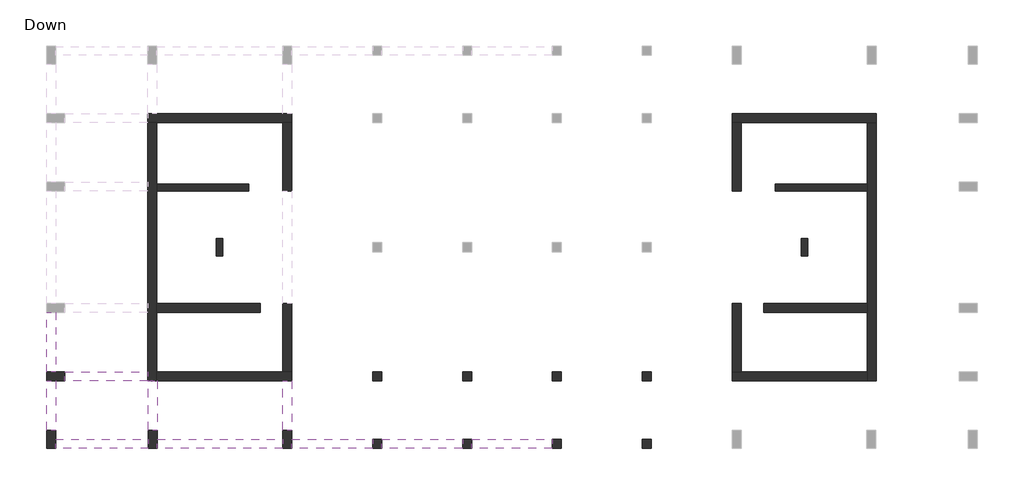
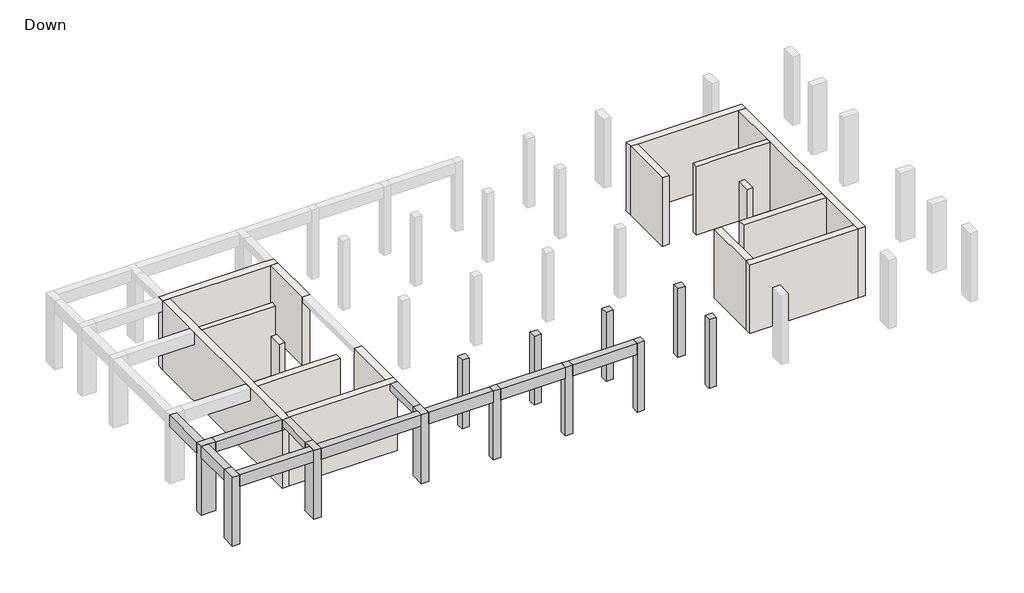
# One storey, part 1 of 2: 16 walls, 12 columns, 10 beams.
"""IFC4 building model written with IfcOpenShell, lengths in millimetres."""

from ifc_helpers import new_model, si_unit, frame, origin, origin_with_axes, place, context, project, spatial, polyline, outline, extrude, faceted_brep, element, save

model = new_model("IFC4")

# Units and contexts
model_context = context("Model", 3, world=origin())
ifc_project = project(units=[si_unit("LENGTHUNIT", "METRE", prefix="MILLI")], contexts=[model_context])

# Site, building, storey
site = spatial("IfcSite", under=ifc_project)
building = spatial("IfcBuilding", under=site)
storey = spatial("IfcBuildingStorey", under=building, Name="Down", Elevation=0.0)

# Beams
placement = place(None, origin())
element("IfcBeam", 1, ObjectType="Concrete Rectengular Beam : 40/40", at=placement, inside=storey, context=model_context, shape_type="Brep", body=[
    faceted_brep([(-15791.2573041, -5152.7195656, 4000.0), (-15391.2573041, -5152.7195656, 4000.0), (-15391.2573041, -2970.6647062, 4000.0), (-15412.8227448, -2970.6647062, 4000.0), (-15591.2573041, -2970.6647062, 4000.0), (-15591.2573041, -2974.5007845, 4000.0), (-15791.2573041, -2974.5007845, 4000.0), (-15391.2573041, -5152.7195656, 3600.0), (-15391.2573041, -2970.6647062, 3600.0), (-15391.2573041, -2970.6647062, 3850.0), (-15791.2573041, -5152.7195656, 3600.0), (-15791.2573041, -2974.5007845, 3600.0), (-15591.2573041, -2974.5007845, 3600.0), (-15591.2573041, -2970.6647062, 3600.0), (-15791.2573041, -2974.5007845, 3850.0)], [[[0, 1, 2, 3, 4, 5, 6]], [[1, 7, 8, 9, 2]], [[7, 10, 11, 12, 13, 8]], [[10, 0, 6, 14, 11]], [[1, 0, 10, 7]], [[2, 9, 8, 13, 4, 3]], [[5, 12, 11, 14, 6]], [[12, 5, 4, 13]]]),
])
element("IfcBeam", 2, ObjectType="Concrete Rectengular Beam : 40/40", at=placement, inside=storey, context=model_context, shape_type="Brep", body=[
    faceted_brep([(-9870.3374688, -5152.7195656, 4000.0), (-9470.3374688, -5152.7195656, 4000.0), (-9470.3374688, -2970.6647062, 4000.0), (-9870.3374688, -2970.6647062, 4000.0), (-9470.3374688, -5152.7195656, 3600.0), (-9470.3374688, -2970.6647062, 3600.0), (-9870.3374688, -5152.7195656, 3600.0), (-9870.3374688, -2970.6647062, 3600.0), (-9870.3374688, -2970.6647062, 3850.0)], [[[0, 1, 2, 3]], [[1, 4, 5, 2]], [[4, 6, 7, 5]], [[6, 0, 3, 8, 7]], [[1, 0, 6, 4]], [[3, 2, 5, 7, 8]]]),
])
element("IfcBeam", 3, ObjectType="Concrete Rectengular Beam : 40/60", at=placement, inside=storey, context=model_context, shape_type="Brep", body=[
    faceted_brep([(-19471.2573041, -2974.5007845, 4000.0), (-15791.2573041, -2974.5007845, 4000.0), (-15591.2573041, -2974.5007845, 4000.0), (-15591.2573041, -2970.6647062, 4000.0), (-15812.8227448, -2970.6647062, 4000.0), (-15812.8227448, -2574.5007845, 4000.0), (-19471.2573041, -2574.5007845, 4000.0), (-19471.2573041, -2974.5007845, 3400.0), (-15591.2573041, -2974.5007845, 3400.0), (-15591.2573041, -2974.5007845, 3600.0), (-19471.2573041, -2574.5007845, 3400.0), (-15812.8227448, -2574.5007845, 3400.0), (-15812.8227448, -2970.6647062, 3400.0), (-15591.2573041, -2970.6647062, 3400.0), (-15812.8227448, -2574.5007845, 3850.0), (-15591.2573041, -2970.6647062, 3600.0)], [[[0, 1, 2, 3, 4, 5, 6]], [[2, 1, 0, 7, 8, 9]], [[8, 7, 10, 11, 12, 13]], [[10, 6, 5, 14, 11]], [[0, 6, 10, 7]], [[4, 12, 11, 14, 5]], [[12, 4, 3, 15, 13]], [[2, 9, 8, 13, 15, 3]]]),
])
element("IfcBeam", 4, ObjectType="Concrete Rectengular Beam : 40/65", at=placement, inside=storey, context=model_context, shape_type="Brep", body=[
    faceted_brep([(-19871.2573041, -5548.8870638, 4000.0), (-19871.2573041, -5948.8870638, 4000.0), (-15791.2573041, -5948.8870638, 4000.0), (-15791.2573041, -5548.8870638, 4000.0), (-19871.2573041, -5948.8870638, 3350.0), (-15791.2573041, -5948.8870638, 3350.0), (-19871.2573041, -5548.8870638, 3350.0), (-15791.2573041, -5548.8870638, 3350.0), (-19871.2573041, -5548.8870638, 3850.0), (-15791.2573041, -5548.8870638, 3850.0)], [[[0, 1, 2, 3]], [[1, 4, 5, 2]], [[4, 6, 7, 5]], [[6, 8, 0, 3, 9, 7]], [[1, 0, 8, 6, 4]], [[3, 2, 5, 7, 9]]]),
])
element("IfcBeam", 5, ObjectType="Concrete Rectengular Beam : 40/65", at=placement, inside=storey, context=model_context, shape_type="Brep", body=[
    faceted_brep([(-15391.2573041, -5548.8870638, 4000.0), (-15391.2573041, -5948.8870638, 4000.0), (-9870.3374688, -5948.8870638, 4000.0), (-9870.3374688, -5548.8870638, 4000.0), (-15391.2573041, -5948.8870638, 3350.0), (-9870.3374688, -5948.8870638, 3350.0), (-15391.2573041, -5548.8870638, 3350.0), (-9870.3374688, -5548.8870638, 3350.0), (-15391.2573041, -5548.8870638, 3850.0), (-9870.3374688, -5548.8870638, 3850.0)], [[[0, 1, 2, 3]], [[1, 4, 5, 2]], [[4, 6, 7, 5]], [[6, 8, 0, 3, 9, 7]], [[1, 0, 8, 6, 4]], [[3, 2, 5, 7, 9]]]),
])
element("IfcBeam", 6, ObjectType="Concrete Rectengular Beam : 40/65", at=placement, inside=storey, context=model_context, shape_type="Brep", body=[
    faceted_brep([(-9470.3374688, -5548.8870638, 4000.0), (-9470.3374688, -5948.8870638, 4000.0), (-5908.6814696, -5948.8870638, 4000.0), (-5908.6814696, -5548.8870638, 4000.0), (-9470.3374688, -5948.8870638, 3350.0), (-5908.6814696, -5948.8870638, 3350.0), (-9470.3374688, -5548.8870638, 3350.0), (-5908.6814696, -5548.8870638, 3350.0), (-9470.3374688, -5548.8870638, 3770.0)], [[[0, 1, 2, 3]], [[1, 4, 5, 2]], [[4, 6, 7, 5]], [[6, 8, 0, 3, 7]], [[1, 0, 8, 6, 4]], [[3, 2, 5, 7]]]),
])
element("IfcBeam", 7, ObjectType="Concrete Rectengular Beam : 40/65", at=placement, inside=storey, context=model_context, shape_type="SweptSolid", body=[
    extrude(outline(polyline([(-1947.0254312, -5548.8870638), (-1947.0254312, -5948.8870638), (-5508.6814696, -5948.8870638), (-5508.6814696, -5548.8870638), (-1947.0254312, -5548.8870638)])), frame((0.0, 0.0, 3350.0), z_axis=(0.0, 0.0, 1.0), x_axis=(1.0, 0.0, 0.0)), (0.0, 0.0, 1.0), 650.0),
])
element("IfcBeam", 8, ObjectType="Concrete Rectengular Beam : 40/65", at=placement, inside=storey, context=model_context, shape_type="Brep", body=[
    faceted_brep([(-19871.2573041, 43.9061014, 4000.0), (-20271.2573041, 43.9061014, 4000.0), (-20271.2573041, -2574.5007845, 4000.0), (-19871.2573041, -2574.5007845, 4000.0), (-20271.2573041, 43.9061014, 3350.0), (-20271.2573041, -2574.5007845, 3350.0), (-19871.2573041, 43.9061014, 3350.0), (-19871.2573041, -2574.5007845, 3350.0), (-19871.2573041, 43.9061014, 3850.0), (-19871.2573041, -2574.5007845, 3850.0)], [[[0, 1, 2, 3]], [[1, 4, 5, 2]], [[4, 6, 7, 5]], [[6, 8, 0, 3, 9, 7]], [[1, 0, 8, 6, 4]], [[3, 2, 5, 7, 9]]]),
])
element("IfcBeam", 9, ObjectType="Concrete Rectengular Beam : 40/65", at=placement, inside=storey, context=model_context, shape_type="Brep", body=[
    faceted_brep([(-19871.2573041, -2974.5007845, 4000.0), (-20271.2573041, -2974.5007845, 4000.0), (-20271.2573041, -5152.7195656, 4000.0), (-19871.2573041, -5152.7195656, 4000.0), (-20271.2573041, -2974.5007845, 3350.0), (-20271.2573041, -5152.7195656, 3350.0), (-19871.2573041, -2974.5007845, 3350.0), (-19871.2573041, -5152.7195656, 3350.0), (-19871.2573041, -2974.5007845, 3850.0)], [[[0, 1, 2, 3]], [[1, 4, 5, 2]], [[4, 6, 7, 5]], [[6, 8, 0, 3, 7]], [[1, 0, 8, 6, 4]], [[3, 2, 5, 7]]]),
])
element("IfcBeam", 10, ObjectType="Concrete Rectengular Beam : 40/65", at=placement, inside=storey, context=model_context, shape_type="SweptSolid", body=[
    extrude(outline(polyline([(-1547.0254312, -5948.8870638), (-1547.0254312, -5548.8870638), (2010.7993238, -5548.8870638), (2010.7993238, -5948.8870638), (-1547.0254312, -5948.8870638)])), frame((0.0, 0.0, 3350.0), z_axis=(0.0, 0.0, 1.0), x_axis=(1.0, 0.0, 0.0)), (0.0, 0.0, 1.0), 650.0),
])

# Columns
element("IfcColumn", 11, ObjectType="Concrete Rectengular Column : 40/40", at=placement, inside=storey, context=model_context, shape_type="Brep", body=[
    faceted_brep([(-5508.6814696, -2574.5007845, 0.0), (-5508.6814696, -2974.5007845, 0.0), (-5908.6814696, -2974.5007845, 0.0), (-5908.6814696, -2574.5007845, 0.0), (-5508.6814696, -2574.5007845, 4000.0), (-5508.6814696, -2974.5007845, 4000.0), (-5508.6814696, -2974.5007845, 3770.0), (-5508.6814696, -2574.5007845, 3770.0), (-5908.6814696, -2974.5007845, 4000.0), (-5908.6814696, -2974.5007845, 3770.0), (-5908.6814696, -2574.5007845, 4000.0), (-5908.6814696, -2574.5007845, 3770.0)], [[[0, 1, 2, 3]], [[4, 5, 6, 1, 0, 7]], [[5, 8, 9, 2, 1, 6]], [[8, 10, 11, 3, 2, 9]], [[10, 4, 7, 0, 3, 11]], [[4, 10, 8, 5]]]),
])
element("IfcColumn", 12, ObjectType="Concrete Rectengular Column : 40/40", at=placement, inside=storey, context=model_context, shape_type="Brep", body=[
    faceted_brep([(-1547.0254312, -2574.5007845, 0.0), (-1547.0254312, -2974.5007845, 0.0), (-1947.0254312, -2974.5007845, 0.0), (-1947.0254312, -2574.5007845, 0.0), (-1547.0254312, -2574.5007845, 4000.0), (-1547.0254312, -2974.5007845, 4000.0), (-1547.0254312, -2974.5007845, 3770.0), (-1547.0254312, -2574.5007845, 3770.0), (-1947.0254312, -2974.5007845, 4000.0), (-1947.0254312, -2974.5007845, 3770.0), (-1947.0254312, -2574.5007845, 4000.0), (-1947.0254312, -2574.5007845, 3770.0)], [[[0, 1, 2, 3]], [[4, 5, 6, 1, 0, 7]], [[5, 8, 9, 2, 1, 6]], [[8, 10, 11, 3, 2, 9]], [[10, 4, 7, 0, 3, 11]], [[4, 10, 8, 5]]]),
])
element("IfcColumn", 13, ObjectType="Concrete Rectengular Column : 40/40", at=placement, inside=storey, context=model_context, shape_type="SweptSolid", body=[
    extrude(outline(polyline([(-1547.0254312, -5548.8870638), (-1547.0254312, -5948.8870638), (-1947.0254312, -5948.8870638), (-1947.0254312, -5548.8870638), (-1547.0254312, -5548.8870638)])), origin_with_axes(), (0.0, 0.0, 1.0), 4000.0),
])
element("IfcColumn", 14, ObjectType="Concrete Rectengular Column : 40/40", at=placement, inside=storey, context=model_context, shape_type="SweptSolid", body=[
    extrude(outline(polyline([(-5508.6814696, -5548.8870638), (-5508.6814696, -5948.8870638), (-5908.6814696, -5948.8870638), (-5908.6814696, -5548.8870638), (-5508.6814696, -5548.8870638)])), origin_with_axes(), (0.0, 0.0, 1.0), 4000.0),
])
element("IfcColumn", 15, ObjectType="Concrete Rectengular Column : 40/40", at=placement, inside=storey, context=model_context, shape_type="Brep", body=[
    faceted_brep([(5972.4553623, -2574.5007845, 0.0), (6372.4553623, -2574.5007845, 0.0), (6372.4553623, -2974.5007845, 0.0), (5972.4553623, -2974.5007845, 0.0), (5972.4553623, -2574.5007845, 4000.0), (5972.4553623, -2574.5007845, 3770.0), (5972.4553623, -2974.5007845, 3770.0), (5972.4553623, -2974.5007845, 4000.0), (6372.4553623, -2974.5007845, 3770.0), (6372.4553623, -2974.5007845, 4000.0), (6372.4553623, -2574.5007845, 3770.0), (6372.4553623, -2574.5007845, 4000.0)], [[[0, 1, 2, 3]], [[4, 5, 0, 3, 6, 7]], [[7, 6, 3, 2, 8, 9]], [[9, 8, 2, 1, 10, 11]], [[11, 10, 1, 0, 5, 4]], [[4, 7, 9, 11]]]),
])
element("IfcColumn", 16, ObjectType="Concrete Rectengular Column : 40/40", at=placement, inside=storey, context=model_context, shape_type="Brep", body=[
    faceted_brep([(2010.7993238, -2574.5007845, 0.0), (2410.7993238, -2574.5007845, 0.0), (2410.7993238, -2974.5007845, 0.0), (2010.7993238, -2974.5007845, 0.0), (2010.7993238, -2574.5007845, 4000.0), (2010.7993238, -2574.5007845, 3770.0), (2010.7993238, -2974.5007845, 3770.0), (2010.7993238, -2974.5007845, 4000.0), (2410.7993238, -2974.5007845, 3770.0), (2410.7993238, -2974.5007845, 4000.0), (2410.7993238, -2574.5007845, 3770.0), (2410.7993238, -2574.5007845, 4000.0)], [[[0, 1, 2, 3]], [[4, 5, 0, 3, 6, 7]], [[7, 6, 3, 2, 8, 9]], [[9, 8, 2, 1, 10, 11]], [[11, 10, 1, 0, 5, 4]], [[4, 7, 9, 11]]]),
])
element("IfcColumn", 17, ObjectType="Concrete Rectengular Column : 40/40", at=placement, inside=storey, context=model_context, shape_type="SweptSolid", body=[
    extrude(outline(polyline([(2010.7993238, -5548.8870638), (2410.7993238, -5548.8870638), (2410.7993238, -5948.8870638), (2010.7993238, -5948.8870638), (2010.7993238, -5548.8870638)])), origin_with_axes(), (0.0, 0.0, 1.0), 4000.0),
])
element("IfcColumn", 18, ObjectType="Concrete Rectengular Column : 40/40", at=placement, inside=storey, context=model_context, shape_type="SweptSolid", body=[
    extrude(outline(polyline([(5972.4553623, -5548.8870638), (6372.4553623, -5548.8870638), (6372.4553623, -5948.8870638), (5972.4553623, -5948.8870638), (5972.4553623, -5548.8870638)])), origin_with_axes(), (0.0, 0.0, 1.0), 4000.0),
])
element("IfcColumn", 19, ObjectType="Concrete Rectengular Column : 40/80", at=placement, inside=storey, context=model_context, shape_type="Brep", body=[
    faceted_brep([(-20271.2573041, -2574.5007845, 0.0), (-19471.2573041, -2574.5007845, 0.0), (-19471.2573041, -2974.5007845, 0.0), (-20271.2573041, -2974.5007845, 0.0), (-20271.2573041, -2574.5007845, 4000.0), (-19871.2573041, -2574.5007845, 4000.0), (-19471.2573041, -2574.5007845, 4000.0), (-19471.2573041, -2974.5007845, 4000.0), (-19871.2573041, -2974.5007845, 4000.0), (-20271.2573041, -2974.5007845, 4000.0)], [[[0, 1, 2, 3]], [[4, 5, 6, 1, 0]], [[6, 7, 2, 1]], [[7, 8, 9, 3, 2]], [[9, 4, 0, 3]], [[4, 9, 8, 7, 6, 5]]]),
])
element("IfcColumn", 20, ObjectType="Concrete Rectengular Column : 40/80", at=placement, inside=storey, context=model_context, shape_type="Brep", body=[
    faceted_brep([(-19871.2573041, -5152.7195656, 0.0), (-19871.2573041, -5952.7195656, 0.0), (-20271.2573041, -5952.7195656, 0.0), (-20271.2573041, -5152.7195656, 0.0), (-19871.2573041, -5152.7195656, 4000.0), (-19871.2573041, -5548.8870638, 4000.0), (-19871.2573041, -5952.7195656, 4000.0), (-20271.2573041, -5952.7195656, 4000.0), (-20271.2573041, -5152.7195656, 4000.0)], [[[0, 1, 2, 3]], [[4, 5, 6, 1, 0]], [[6, 7, 2, 1]], [[7, 8, 3, 2]], [[8, 4, 0, 3]], [[4, 8, 7, 6, 5]]]),
])
element("IfcColumn", 21, ObjectType="Concrete Rectengular Column : 40/80", at=placement, inside=storey, context=model_context, shape_type="Brep", body=[
    faceted_brep([(-15391.2573041, -5152.7195656, 0.0), (-15391.2573041, -5952.7195656, 0.0), (-15791.2573041, -5952.7195656, 0.0), (-15791.2573041, -5152.7195656, 0.0), (-15391.2573041, -5152.7195656, 4000.0), (-15391.2573041, -5548.8870638, 4000.0), (-15391.2573041, -5952.7195656, 4000.0), (-15791.2573041, -5952.7195656, 4000.0), (-15791.2573041, -5548.8870638, 4000.0), (-15791.2573041, -5152.7195656, 4000.0)], [[[0, 1, 2, 3]], [[4, 5, 6, 1, 0]], [[6, 7, 2, 1]], [[7, 8, 9, 3, 2]], [[9, 4, 0, 3]], [[4, 9, 8, 7, 6, 5]]]),
])
element("IfcColumn", 22, ObjectType="Concrete Rectengular Column : 40/80", at=placement, inside=storey, context=model_context, shape_type="Brep", body=[
    faceted_brep([(-9470.3374688, -5152.7195656, 0.0), (-9470.3374688, -5952.7195656, 0.0), (-9870.3374688, -5952.7195656, 0.0), (-9870.3374688, -5152.7195656, 0.0), (-9470.3374688, -5152.7195656, 4000.0), (-9470.3374688, -5548.8870638, 4000.0), (-9470.3374688, -5952.7195656, 4000.0), (-9870.3374688, -5952.7195656, 4000.0), (-9870.3374688, -5548.8870638, 4000.0), (-9870.3374688, -5152.7195656, 4000.0)], [[[0, 1, 2, 3]], [[4, 5, 6, 1, 0]], [[6, 7, 2, 1]], [[7, 8, 9, 3, 2]], [[9, 4, 0, 3]], [[4, 9, 8, 7, 6, 5]]]),
])

# Walls
element("IfcWall", 23, ObjectType="30", at=placement, inside=storey, context=model_context, shape_type="Brep", body=[
    faceted_brep([(-15412.8227448, 5394.6720806, 0.0), (-11354.3869672, 5394.6720806, 0.0), (-11354.3869672, 5394.6720806, 3770.0), (-11354.3869672, 5394.6720806, 4000.0), (-12794.417038, 5394.6720806, 4000.0), (-15412.8227448, 5394.6720806, 4000.0), (-15412.8227448, 5694.6720806, 0.0), (-15412.8227448, 5694.6720806, 4000.0), (-11354.3869672, 5694.6720806, 4000.0), (-11354.3869672, 5694.6720806, 0.0)], [[[0, 1, 2, 3, 4, 5]], [[6, 7, 8, 9]], [[1, 0, 6, 9]], [[3, 2, 1, 9, 8]], [[5, 4, 3, 8, 7]], [[0, 5, 7, 6]]]),
])
element("IfcWall", 24, ObjectType="30", at=placement, inside=storey, context=model_context, shape_type="Brep", body=[
    faceted_brep([(-12798.865318, 3298.8134973, 0.0), (-12798.865318, 2525.3463223, 0.0), (-12798.865318, 2525.3463223, 4000.0), (-12798.865318, 3298.8134973, 4000.0), (-12498.865318, 3298.8134973, 0.0), (-12498.865318, 3298.8134973, 3770.0), (-12498.865318, 3298.8134973, 4000.0), (-12498.865318, 2525.3463223, 4000.0), (-12498.865318, 2525.3463223, 3770.0), (-12498.865318, 2525.3463223, 0.0), (-12794.417038, 2525.3463223, 4000.0), (-12794.417038, 3298.8134973, 4000.0)], [[[0, 1, 2, 3]], [[4, 5, 6, 7, 8, 9]], [[1, 0, 4, 9]], [[2, 1, 9, 8, 7, 10]], [[3, 2, 10, 7, 6, 11]], [[0, 3, 11, 6, 5, 4]]]),
])
element("IfcWall", 25, ObjectType="30", at=placement, inside=storey, context=model_context, shape_type="Brep", body=[
    faceted_brep([(15876.5966375, 5694.6720806, 0.0), (11818.1608598, 5694.6720806, 0.0), (11818.1608598, 5694.6720806, 4000.0), (15876.5966375, 5694.6720806, 4000.0), (15876.5966375, 5394.6720806, 0.0), (15876.5966375, 5394.6720806, 4000.0), (13258.1909307, 5394.6720806, 4000.0), (11818.1608598, 5394.6720806, 4000.0), (11818.1608598, 5394.6720806, 3770.0), (11818.1608598, 5394.6720806, 0.0)], [[[0, 1, 2, 3]], [[4, 5, 6, 7, 8, 9]], [[1, 0, 4, 9]], [[2, 1, 9, 8, 7]], [[3, 2, 7, 6, 5]], [[0, 3, 5, 4]]]),
])
element("IfcWall", 26, ObjectType="30", at=placement, inside=storey, context=model_context, shape_type="Brep", body=[
    faceted_brep([(12962.6392106, 3298.8134973, 0.0), (12962.6392106, 2525.3463223, 0.0), (12962.6392106, 2525.3463223, 3770.0), (12962.6392106, 2525.3463223, 4000.0), (12962.6392106, 3298.8134973, 4000.0), (12962.6392106, 3298.8134973, 3770.0), (13262.6392106, 3298.8134973, 0.0), (13262.6392106, 3298.8134973, 4000.0), (13262.6392106, 2525.3463223, 4000.0), (13262.6392106, 2525.3463223, 0.0), (13258.1909307, 2525.3463223, 4000.0), (13258.1909307, 3298.8134973, 4000.0)], [[[0, 1, 2, 3, 4, 5]], [[6, 7, 8, 9]], [[1, 0, 6, 9]], [[3, 2, 1, 9, 8, 10]], [[4, 3, 10, 8, 7, 11]], [[0, 5, 4, 11, 7, 6]]]),
])
element("IfcWall", 27, ObjectType="40", at=placement, inside=storey, context=model_context, shape_type="Brep", body=[
    faceted_brep([(-15812.8227448, 8413.6899891, 0.0), (-15412.8227448, 8413.6899891, 0.0), (-9870.3374688, 8413.6899891, 0.0), (-9470.3374688, 8413.6899891, 0.0), (-9470.3374688, 8413.6899891, 4000.0), (-9870.3374688, 8413.6899891, 4000.0), (-11354.3869672, 8413.6899891, 4000.0), (-15412.8227448, 8413.6899891, 4000.0), (-15812.8227448, 8413.6899891, 4000.0), (-15812.8227448, 8413.6899891, 3400.0), (-15812.8227448, 8813.6899891, 0.0), (-15812.8227448, 8813.6899891, 3400.0), (-15812.8227448, 8813.6899891, 3600.0), (-15812.8227448, 8813.6899891, 4000.0), (-15412.8227448, 8813.6899891, 4000.0), (-9870.3374688, 8813.6899891, 4000.0), (-9470.3374688, 8813.6899891, 4000.0), (-9470.3374688, 8813.6899891, 3600.0), (-9470.3374688, 8813.6899891, 0.0)], [[[0, 1, 2, 3, 4, 5, 6, 7, 8, 9]], [[10, 11, 12, 13, 14, 15, 16, 17, 18]], [[3, 2, 1, 0, 10, 18]], [[8, 7, 6, 5, 4, 16, 15, 14, 13]], [[4, 3, 18, 17, 16]], [[0, 9, 8, 13, 12, 11, 10]]]),
])
element("IfcWall", 28, ObjectType="40", at=placement, inside=storey, context=model_context, shape_type="Brep", body=[
    faceted_brep([(-9870.3374688, 8413.6899891, 0.0), (-9870.3374688, 5392.831899, 0.0), (-9870.3374688, 5392.831899, 3700.0), (-9870.3374688, 5392.831899, 4000.0), (-9870.3374688, 8413.6899891, 4000.0), (-9870.3374688, 8413.6899891, 3770.0), (-9470.3374688, 8413.6899891, 0.0), (-9470.3374688, 8413.6899891, 4000.0), (-9470.3374688, 5392.831899, 4000.0), (-9470.3374688, 5392.831899, 3700.0), (-9470.3374688, 5392.831899, 0.0)], [[[0, 1, 2, 3, 4, 5]], [[6, 7, 8, 9, 10]], [[1, 0, 6, 10]], [[3, 2, 1, 10, 9, 8]], [[4, 3, 8, 7]], [[0, 5, 4, 7, 6]]]),
])
element("IfcWall", 29, ObjectType="40", at=placement, inside=storey, context=model_context, shape_type="Brep", body=[
    faceted_brep([(-15812.8227448, 8413.6899891, 0.0), (-15812.8227448, -2970.6647062, 0.0), (-15812.8227448, -2970.6647062, 3400.0), (-15812.8227448, -2970.6647062, 4000.0), (-15812.8227448, -2574.5007845, 4000.0), (-15812.8227448, 43.9061014, 4000.0), (-15812.8227448, 443.9061014, 4000.0), (-15812.8227448, 5388.9969998, 4000.0), (-15812.8227448, 5788.9969998, 4000.0), (-15812.8227448, 8413.6899891, 4000.0), (-15812.8227448, 8413.6899891, 3850.0), (-15412.8227448, 8413.6899891, 0.0), (-15412.8227448, 8413.6899891, 4000.0), (-15412.8227448, 5694.6720806, 4000.0), (-15412.8227448, 5394.6720806, 4000.0), (-15412.8227448, 443.9061014, 4000.0), (-15412.8227448, 43.9061014, 4000.0), (-15412.8227448, -2570.6647062, 4000.0), (-15412.8227448, -2970.6647062, 4000.0), (-15412.8227448, -2970.6647062, 0.0), (-15412.8227448, -2570.6647062, 0.0), (-15412.8227448, 43.9061014, 0.0), (-15412.8227448, 443.9061014, 0.0), (-15412.8227448, 5394.6720806, 0.0), (-15412.8227448, 5694.6720806, 0.0), (-15591.2573041, -2970.6647062, 4000.0)], [[[0, 1, 2, 3, 4, 5, 6, 7, 8, 9, 10]], [[11, 12, 13, 14, 15, 16, 17, 18, 19, 20, 21, 22, 23, 24]], [[1, 0, 11, 24, 23, 22, 21, 20, 19]], [[9, 8, 7, 6, 5, 4, 3, 25, 18, 17, 16, 15, 14, 13, 12]], [[0, 10, 9, 12, 11]], [[3, 2, 1, 19, 18, 25]]]),
])
element("IfcWall", 30, ObjectType="40", at=placement, inside=storey, context=model_context, shape_type="Brep", body=[
    faceted_brep([(-15412.8227448, -2970.6647062, 0.0), (-9470.3374688, -2970.6647062, 0.0), (-9470.3374688, -2970.6647062, 3600.0), (-9470.3374688, -2970.6647062, 4000.0), (-9870.3374688, -2970.6647062, 4000.0), (-15391.2573041, -2970.6647062, 4000.0), (-15412.8227448, -2970.6647062, 4000.0), (-15412.8227448, -2570.6647062, 0.0), (-15412.8227448, -2570.6647062, 3770.0), (-15412.8227448, -2570.6647062, 4000.0), (-9870.3374688, -2570.6647062, 4000.0), (-9470.3374688, -2570.6647062, 4000.0), (-9470.3374688, -2570.6647062, 0.0), (-9870.3374688, -2570.6647062, 0.0)], [[[0, 1, 2, 3, 4, 5, 6]], [[7, 8, 9, 10, 11, 12, 13]], [[1, 0, 7, 13, 12]], [[6, 5, 4, 3, 11, 10, 9]], [[0, 6, 9, 8, 7]], [[3, 2, 1, 12, 11]]]),
])
element("IfcWall", 31, ObjectType="40", at=placement, inside=storey, context=model_context, shape_type="Brep", body=[
    faceted_brep([(-9470.3374688, -2570.6647062, 0.0), (-9470.3374688, 443.9061014, 0.0), (-9470.3374688, 443.9061014, 3700.0), (-9470.3374688, 443.9061014, 4000.0), (-9470.3374688, -2570.6647062, 4000.0), (-9870.3374688, -2570.6647062, 0.0), (-9870.3374688, -2570.6647062, 3770.0), (-9870.3374688, -2570.6647062, 4000.0), (-9870.3374688, 443.9061014, 4000.0), (-9870.3374688, 443.9061014, 3700.0), (-9870.3374688, 443.9061014, 0.0)], [[[0, 1, 2, 3, 4]], [[5, 6, 7, 8, 9, 10]], [[1, 0, 5, 10]], [[3, 2, 1, 10, 9, 8]], [[4, 3, 8, 7]], [[0, 4, 7, 6, 5]]]),
])
element("IfcWall", 32, ObjectType="40", at=placement, inside=storey, context=model_context, shape_type="Brep", body=[
    faceted_brep([(-10863.8957288, 443.9061014, 0.0), (-15412.8227448, 443.9061014, 0.0), (-15412.8227448, 443.9061014, 4000.0), (-12794.417038, 443.9061014, 4000.0), (-10863.8957288, 443.9061014, 4000.0), (-10863.8957288, 443.9061014, 3770.0), (-10863.8957288, 43.9061014, 0.0), (-10863.8957288, 43.9061014, 3770.0), (-10863.8957288, 43.9061014, 4000.0), (-15412.8227448, 43.9061014, 4000.0), (-15412.8227448, 43.9061014, 3770.0), (-15412.8227448, 43.9061014, 0.0)], [[[0, 1, 2, 3, 4, 5]], [[6, 7, 8, 9, 10, 11]], [[1, 0, 6, 11]], [[4, 3, 2, 9, 8]], [[0, 5, 4, 8, 7, 6]], [[2, 1, 11, 10, 9]]]),
])
element("IfcWall", 33, ObjectType="40", at=placement, inside=storey, context=model_context, shape_type="Brep", body=[
    faceted_brep([(16276.5966375, 8813.6899891, 0.0), (9934.1113614, 8813.6899891, 0.0), (9934.1113614, 8813.6899891, 3600.0), (9934.1113614, 8813.6899891, 4000.0), (10334.1113614, 8813.6899891, 4000.0), (15876.5966375, 8813.6899891, 4000.0), (16276.5966375, 8813.6899891, 4000.0), (16276.5966375, 8813.6899891, 3600.0), (16276.5966375, 8813.6899891, 3400.0), (16276.5966375, 8413.6899891, 0.0), (16276.5966375, 8413.6899891, 3400.0), (16276.5966375, 8413.6899891, 4000.0), (15876.5966375, 8413.6899891, 4000.0), (11818.1608598, 8413.6899891, 4000.0), (10334.1113614, 8413.6899891, 4000.0), (9934.1113614, 8413.6899891, 4000.0), (9934.1113614, 8413.6899891, 0.0), (10334.1113614, 8413.6899891, 0.0), (15876.5966375, 8413.6899891, 0.0)], [[[0, 1, 2, 3, 4, 5, 6, 7, 8]], [[9, 10, 11, 12, 13, 14, 15, 16, 17, 18]], [[1, 0, 9, 18, 17, 16]], [[6, 5, 4, 3, 15, 14, 13, 12, 11]], [[3, 2, 1, 16, 15]], [[0, 8, 7, 6, 11, 10, 9]]]),
])
element("IfcWall", 34, ObjectType="40", at=placement, inside=storey, context=model_context, shape_type="Brep", body=[
    faceted_brep([(9934.1113614, 8413.6899891, 0.0), (9934.1113614, 5392.831899, 0.0), (9934.1113614, 5392.831899, 3700.0), (9934.1113614, 5392.831899, 4000.0), (9934.1113614, 8413.6899891, 4000.0), (10334.1113614, 8413.6899891, 0.0), (10334.1113614, 8413.6899891, 3770.0), (10334.1113614, 8413.6899891, 4000.0), (10334.1113614, 5392.831899, 4000.0), (10334.1113614, 5392.831899, 3700.0), (10334.1113614, 5392.831899, 0.0)], [[[0, 1, 2, 3, 4]], [[5, 6, 7, 8, 9, 10]], [[1, 0, 5, 10]], [[3, 2, 1, 10, 9, 8]], [[4, 3, 8, 7]], [[0, 4, 7, 6, 5]]]),
])
element("IfcWall", 35, ObjectType="40", at=placement, inside=storey, context=model_context, shape_type="Brep", body=[
    faceted_brep([(15876.5966375, 8413.6899891, 0.0), (15876.5966375, 5694.6720806, 0.0), (15876.5966375, 5394.6720806, 0.0), (15876.5966375, 443.9061014, 0.0), (15876.5966375, 43.9061014, 0.0), (15876.5966375, -2570.6647062, 0.0), (15876.5966375, -2970.6647062, 0.0), (15876.5966375, -2970.6647062, 4000.0), (15876.5966375, -2570.6647062, 4000.0), (15876.5966375, 43.9061014, 4000.0), (15876.5966375, 443.9061014, 4000.0), (15876.5966375, 5394.6720806, 4000.0), (15876.5966375, 5694.6720806, 4000.0), (15876.5966375, 8413.6899891, 4000.0), (16276.5966375, 8413.6899891, 0.0), (16276.5966375, 8413.6899891, 3850.0), (16276.5966375, 8413.6899891, 4000.0), (16276.5966375, 5788.9969998, 4000.0), (16276.5966375, 5388.9969998, 4000.0), (16276.5966375, 443.9061014, 4000.0), (16276.5966375, 43.9061014, 4000.0), (16276.5966375, -2574.5007845, 4000.0), (16276.5966375, -2970.6647062, 4000.0), (16276.5966375, -2970.6647062, 3400.0), (16276.5966375, -2970.6647062, 0.0)], [[[0, 1, 2, 3, 4, 5, 6, 7, 8, 9, 10, 11, 12, 13]], [[14, 15, 16, 17, 18, 19, 20, 21, 22, 23, 24]], [[6, 5, 4, 3, 2, 1, 0, 14, 24]], [[13, 12, 11, 10, 9, 8, 7, 22, 21, 20, 19, 18, 17, 16]], [[0, 13, 16, 15, 14]], [[7, 6, 24, 23, 22]]]),
])
element("IfcWall", 36, ObjectType="40", at=placement, inside=storey, context=model_context, shape_type="Brep", body=[
    faceted_brep([(15876.5966375, -2570.6647062, 0.0), (10334.1113614, -2570.6647062, 0.0), (9934.1113614, -2570.6647062, 0.0), (9934.1113614, -2570.6647062, 4000.0), (10334.1113614, -2570.6647062, 4000.0), (15876.5966375, -2570.6647062, 4000.0), (15876.5966375, -2570.6647062, 3770.0), (15876.5966375, -2970.6647062, 0.0), (15876.5966375, -2970.6647062, 4000.0), (15855.0311968, -2970.6647062, 4000.0), (10334.1113614, -2970.6647062, 4000.0), (9934.1113614, -2970.6647062, 4000.0), (9934.1113614, -2970.6647062, 3600.0), (9934.1113614, -2970.6647062, 0.0)], [[[0, 1, 2, 3, 4, 5, 6]], [[7, 8, 9, 10, 11, 12, 13]], [[2, 1, 0, 7, 13]], [[5, 4, 3, 11, 10, 9, 8]], [[0, 6, 5, 8, 7]], [[3, 2, 13, 12, 11]]]),
])
element("IfcWall", 37, ObjectType="40", at=placement, inside=storey, context=model_context, shape_type="Brep", body=[
    faceted_brep([(10334.1113614, -2570.6647062, 0.0), (10334.1113614, 443.9061014, 0.0), (10334.1113614, 443.9061014, 3700.0), (10334.1113614, 443.9061014, 4000.0), (10334.1113614, -2570.6647062, 4000.0), (10334.1113614, -2570.6647062, 3770.0), (9934.1113614, -2570.6647062, 0.0), (9934.1113614, -2570.6647062, 4000.0), (9934.1113614, 443.9061014, 4000.0), (9934.1113614, 443.9061014, 3700.0), (9934.1113614, 443.9061014, 0.0)], [[[0, 1, 2, 3, 4, 5]], [[6, 7, 8, 9, 10]], [[1, 0, 6, 10]], [[3, 2, 1, 10, 9, 8]], [[4, 3, 8, 7]], [[0, 5, 4, 7, 6]]]),
])
element("IfcWall", 38, ObjectType="40", at=placement, inside=storey, context=model_context, shape_type="Brep", body=[
    faceted_brep([(11327.6696215, 43.9061014, 0.0), (15876.5966375, 43.9061014, 0.0), (15876.5966375, 43.9061014, 3770.0), (15876.5966375, 43.9061014, 4000.0), (11327.6696215, 43.9061014, 4000.0), (11327.6696215, 43.9061014, 3770.0), (11327.6696215, 443.9061014, 0.0), (11327.6696215, 443.9061014, 3770.0), (11327.6696215, 443.9061014, 4000.0), (13258.1909307, 443.9061014, 4000.0), (15876.5966375, 443.9061014, 4000.0), (15876.5966375, 443.9061014, 0.0)], [[[0, 1, 2, 3, 4, 5]], [[6, 7, 8, 9, 10, 11]], [[1, 0, 6, 11]], [[4, 3, 10, 9, 8]], [[0, 5, 4, 8, 7, 6]], [[3, 2, 1, 11, 10]]]),
])

save(model, "model.ifc")

# Revit data of these elements
# Project information
#   Project Issue Date = "Issue Date"
#   Project Status = "Project Status"
#   Client Name = "לקוח"
#   Project Address = "Enter address here"
#   Project Name = "Project 048"
#   Project Number = "מספר פרויקט"
# Type "Concrete Rectengular Beam : 40/40"
#   Length [instance default] = 152.4 cm
#   b = 40 cm
#   h = 40 cm
#   Structural Material [instance default] = Concrete
#   Assembly Code = ""
# Type "Concrete Rectengular Beam : 40/60"
#   Length [instance default] = 152.4 cm
#   b = 40 cm
#   h = 60 cm
#   Structural Material [instance default] = Concrete
#   Assembly Code = ""
# Type "Concrete Rectengular Beam : 40/65"
#   Length [instance default] = 152.4 cm
#   b = 40 cm
#   h = 65 cm
#   Structural Material [instance default] = Concrete
#   Assembly Code = ""
# Type "Concrete Rectengular Column : 40/40"
#   b = 40 cm
#   h = 40 cm
#   Structural Material [instance default] = Concrete
# Type "Concrete Rectengular Column : 40/80"
#   b = 40 cm
#   h = 80 cm
#   Structural Material [instance default] = Concrete
# Type "30"
#   Layers, outside or top first: 30 cm "Concrete" (function 1)
# Type "40"
#   Layers, outside or top first: 40 cm "Concrete" (function 1)
# Element 1 (IfcBeam, "Concrete Rectengular Beam : 40/40")
#   Comments = ""
#   Mark = "B3"
#   SOFiSTiK_AMG_Comments = ""
#   SOFiSTiK_AMG_Scheduled = yes
#   SOFiSTiK_AMG_Adjusted = yes
#   Structural Material = Concrete
#   Phase Created = New Construction
#   Materials on its faces: "Concrete"
# Element 2 (IfcBeam, "Concrete Rectengular Beam : 40/40")
#   Comments = ""
#   Mark = "B4"
#   SOFiSTiK_AMG_Comments = ""
#   SOFiSTiK_AMG_Scheduled = yes
#   SOFiSTiK_AMG_Adjusted = yes
#   Structural Material = Concrete
#   Phase Created = New Construction
#   Materials on its faces: "Concrete"
# Element 3 (IfcBeam, "Concrete Rectengular Beam : 40/60")
#   Comments = ""
#   Mark = "B12"
#   SOFiSTiK_AMG_Comments = ""
#   SOFiSTiK_AMG_Scheduled = yes
#   SOFiSTiK_AMG_Adjusted = yes
#   Structural Material = Concrete
#   Phase Created = New Construction
#   Materials on its faces: "Concrete"
# Element 4 (IfcBeam, "Concrete Rectengular Beam : 40/65")
#   Comments = ""
#   Mark = "B17"
#   SOFiSTiK_AMG_Comments = ""
#   SOFiSTiK_AMG_Scheduled = yes
#   SOFiSTiK_AMG_Adjusted = yes
#   Structural Material = Concrete
#   Phase Created = New Construction
#   Materials on its faces: "Concrete"
# Element 5 (IfcBeam, "Concrete Rectengular Beam : 40/65")
#   Comments = ""
#   Mark = "B18"
#   SOFiSTiK_AMG_Comments = ""
#   SOFiSTiK_AMG_Scheduled = yes
#   SOFiSTiK_AMG_Adjusted = yes
#   Structural Material = Concrete
#   Phase Created = New Construction
#   Materials on its faces: "Concrete"
# Element 6 (IfcBeam, "Concrete Rectengular Beam : 40/65")
#   Comments = ""
#   Mark = "B21"
#   SOFiSTiK_AMG_Comments = ""
#   SOFiSTiK_AMG_Scheduled = yes
#   SOFiSTiK_AMG_Adjusted = yes
#   Structural Material = Concrete
#   Phase Created = New Construction
#   Materials on its faces: "Concrete"
# Element 7 (IfcBeam, "Concrete Rectengular Beam : 40/65")
#   Comments = ""
#   Mark = "B22"
#   SOFiSTiK_AMG_Comments = ""
#   SOFiSTiK_AMG_Scheduled = yes
#   SOFiSTiK_AMG_Adjusted = yes
#   Structural Material = Concrete
#   Phase Created = New Construction
#   Materials on its faces: "Concrete"
# Element 8 (IfcBeam, "Concrete Rectengular Beam : 40/65")
#   Comments = ""
#   Mark = "B26"
#   SOFiSTiK_AMG_Comments = ""
#   SOFiSTiK_AMG_Scheduled = yes
#   SOFiSTiK_AMG_Adjusted = yes
#   Structural Material = Concrete
#   Phase Created = New Construction
#   Materials on its faces: "Concrete"
# Element 9 (IfcBeam, "Concrete Rectengular Beam : 40/65")
#   Comments = ""
#   Mark = "B27"
#   SOFiSTiK_AMG_Comments = ""
#   SOFiSTiK_AMG_Scheduled = yes
#   SOFiSTiK_AMG_Adjusted = yes
#   Structural Material = Concrete
#   Phase Created = New Construction
#   Materials on its faces: "Concrete"
# Element 10 (IfcBeam, "Concrete Rectengular Beam : 40/65")
#   Comments = ""
#   Mark = "B42"
#   SOFiSTiK_AMG_Comments = ""
#   SOFiSTiK_AMG_Scheduled = yes
#   SOFiSTiK_AMG_Adjusted = yes
#   Structural Material = Concrete
#   Phase Created = New Construction
#   Materials on its faces: "Concrete"
# Element 11 (IfcColumn, "Concrete Rectengular Column : 40/40")
#   Comments = ""
#   Mark = "C5"
#   SOFiSTiK_AMG_Comments = ""
#   SOFiSTiK_AMG_Scheduled = yes
#   SOFiSTiK_AMG_Adjusted = yes
#   Structural Material = Concrete
#   Phase Created = New Construction
#   Materials on its faces: "Concrete"
# Element 12 (IfcColumn, "Concrete Rectengular Column : 40/40")
#   Comments = ""
#   Mark = "C6"
#   SOFiSTiK_AMG_Comments = ""
#   SOFiSTiK_AMG_Scheduled = yes
#   SOFiSTiK_AMG_Adjusted = yes
#   Structural Material = Concrete
#   Phase Created = New Construction
#   Materials on its faces: "Concrete"
# Element 13 (IfcColumn, "Concrete Rectengular Column : 40/40")
#   Comments = ""
#   Mark = "C7"
#   SOFiSTiK_AMG_Comments = ""
#   SOFiSTiK_AMG_Scheduled = yes
#   SOFiSTiK_AMG_Adjusted = yes
#   Structural Material = Concrete
#   Phase Created = New Construction
#   Materials on its faces: "Concrete"
# Element 14 (IfcColumn, "Concrete Rectengular Column : 40/40")
#   Comments = ""
#   Mark = "C8"
#   SOFiSTiK_AMG_Comments = ""
#   SOFiSTiK_AMG_Scheduled = yes
#   SOFiSTiK_AMG_Adjusted = yes
#   Structural Material = Concrete
#   Phase Created = New Construction
#   Materials on its faces: "Concrete"
# Element 15 (IfcColumn, "Concrete Rectengular Column : 40/40")
#   Comments = ""
#   Mark = "C15"
#   SOFiSTiK_AMG_Comments = ""
#   SOFiSTiK_AMG_Scheduled = yes
#   SOFiSTiK_AMG_Adjusted = yes
#   Structural Material = Concrete
#   Phase Created = New Construction
#   Materials on its faces: "Concrete"
# Element 16 (IfcColumn, "Concrete Rectengular Column : 40/40")
#   Comments = ""
#   Mark = "C16"
#   SOFiSTiK_AMG_Comments = ""
#   SOFiSTiK_AMG_Scheduled = yes
#   SOFiSTiK_AMG_Adjusted = yes
#   Structural Material = Concrete
#   Phase Created = New Construction
#   Materials on its faces: "Concrete"
# Element 17 (IfcColumn, "Concrete Rectengular Column : 40/40")
#   Comments = ""
#   Mark = "C17"
#   SOFiSTiK_AMG_Comments = ""
#   SOFiSTiK_AMG_Scheduled = yes
#   SOFiSTiK_AMG_Adjusted = yes
#   Structural Material = Concrete
#   Phase Created = New Construction
#   Materials on its faces: "Concrete"
# Element 18 (IfcColumn, "Concrete Rectengular Column : 40/40")
#   Comments = ""
#   Mark = "C18"
#   SOFiSTiK_AMG_Comments = ""
#   SOFiSTiK_AMG_Scheduled = yes
#   SOFiSTiK_AMG_Adjusted = yes
#   Structural Material = Concrete
#   Phase Created = New Construction
#   Materials on its faces: "Concrete"
# Element 19 (IfcColumn, "Concrete Rectengular Column : 40/80")
#   Comments = ""
#   Mark = "C25"
#   SOFiSTiK_AMG_Comments = ""
#   SOFiSTiK_AMG_Scheduled = yes
#   SOFiSTiK_AMG_Adjusted = yes
#   Structural Material = Concrete
#   Phase Created = New Construction
#   Materials on its faces: "Concrete"
# Element 20 (IfcColumn, "Concrete Rectengular Column : 40/80")
#   Comments = ""
#   Mark = "C26"
#   SOFiSTiK_AMG_Comments = ""
#   SOFiSTiK_AMG_Scheduled = yes
#   SOFiSTiK_AMG_Adjusted = yes
#   Structural Material = Concrete
#   Phase Created = New Construction
#   Materials on its faces: "Concrete"
# Element 21 (IfcColumn, "Concrete Rectengular Column : 40/80")
#   Comments = ""
#   Mark = "C27"
#   SOFiSTiK_AMG_Comments = ""
#   SOFiSTiK_AMG_Scheduled = yes
#   SOFiSTiK_AMG_Adjusted = yes
#   Structural Material = Concrete
#   Phase Created = New Construction
#   Materials on its faces: "Concrete"
# Element 22 (IfcColumn, "Concrete Rectengular Column : 40/80")
#   Comments = ""
#   Mark = "C28"
#   SOFiSTiK_AMG_Comments = ""
#   SOFiSTiK_AMG_Scheduled = yes
#   SOFiSTiK_AMG_Adjusted = yes
#   Structural Material = Concrete
#   Phase Created = New Construction
#   Materials on its faces: "Concrete"
# Element 23 (IfcWall, "30")
#   Comments = ""
#   Mark = "W13"
#   SOFiSTiK_AMG_Comments = ""
#   Top Offset = 0 cm
#   Base Offset = 0 cm
#   Unconnected Height = 400 cm
#   wall height = 400 cm
#   SOFiSTiK_AMG_Scheduled = yes
#   SOFiSTiK_AMG_Adjusted = yes
#   Phase Created = New Construction
#   Base Constraint = Down
#   Top Constraint = Typical Floor
#   Materials on its faces: "Concrete"
# Element 24 (IfcWall, "30")
#   Comments = ""
#   Mark = "W14"
#   SOFiSTiK_AMG_Comments = ""
#   Top Offset = 0 cm
#   Base Offset = 0 cm
#   Unconnected Height = 400 cm
#   wall height = 400 cm
#   SOFiSTiK_AMG_Scheduled = yes
#   SOFiSTiK_AMG_Adjusted = yes
#   Phase Created = New Construction
#   Base Constraint = Down
#   Top Constraint = Typical Floor
#   Materials on its faces: "Concrete"
# Element 25 (IfcWall, "30")
#   Comments = ""
#   Mark = "W15"
#   SOFiSTiK_AMG_Comments = ""
#   Top Offset = 0 cm
#   Base Offset = 0 cm
#   Unconnected Height = 400 cm
#   wall height = 400 cm
#   SOFiSTiK_AMG_Scheduled = yes
#   SOFiSTiK_AMG_Adjusted = yes
#   Phase Created = New Construction
#   Base Constraint = Down
#   Top Constraint = Typical Floor
#   Materials on its faces: "Concrete"
# Element 26 (IfcWall, "30")
#   Comments = ""
#   Mark = "W16"
#   SOFiSTiK_AMG_Comments = ""
#   Top Offset = 0 cm
#   Base Offset = 0 cm
#   Unconnected Height = 400 cm
#   wall height = 400 cm
#   SOFiSTiK_AMG_Scheduled = yes
#   SOFiSTiK_AMG_Adjusted = yes
#   Phase Created = New Construction
#   Base Constraint = Down
#   Top Constraint = Typical Floor
#   Materials on its faces: "Concrete"
# Element 27 (IfcWall, "40")
#   Comments = ""
#   Mark = "W1"
#   SOFiSTiK_AMG_Comments = ""
#   Top Offset = 0 cm
#   Base Offset = 0 cm
#   Unconnected Height = 400 cm
#   wall height = 400 cm
#   SOFiSTiK_AMG_Scheduled = yes
#   SOFiSTiK_AMG_Adjusted = yes
#   Phase Created = New Construction
#   Base Constraint = Down
#   Top Constraint = Typical Floor
#   Materials on its faces: "Concrete"
# Element 28 (IfcWall, "40")
#   Comments = ""
#   Mark = "W2"
#   SOFiSTiK_AMG_Comments = ""
#   Top Offset = 0 cm
#   Base Offset = 0 cm
#   Unconnected Height = 400 cm
#   wall height = 400 cm
#   SOFiSTiK_AMG_Scheduled = yes
#   SOFiSTiK_AMG_Adjusted = yes
#   Phase Created = New Construction
#   Base Constraint = Down
#   Top Constraint = Typical Floor
#   Materials on its faces: "Concrete"
# Element 29 (IfcWall, "40")
#   Comments = ""
#   Mark = "W3"
#   SOFiSTiK_AMG_Comments = ""
#   Top Offset = 0 cm
#   Base Offset = 0 cm
#   Unconnected Height = 400 cm
#   wall height = 400 cm
#   SOFiSTiK_AMG_Scheduled = yes
#   SOFiSTiK_AMG_Adjusted = yes
#   Phase Created = New Construction
#   Base Constraint = Down
#   Top Constraint = Typical Floor
#   Materials on its faces: "Concrete"
# Element 30 (IfcWall, "40")
#   Comments = ""
#   Mark = "W4"
#   SOFiSTiK_AMG_Comments = ""
#   Top Offset = 0 cm
#   Base Offset = 0 cm
#   Unconnected Height = 400 cm
#   wall height = 400 cm
#   SOFiSTiK_AMG_Scheduled = yes
#   SOFiSTiK_AMG_Adjusted = yes
#   Phase Created = New Construction
#   Base Constraint = Down
#   Top Constraint = Typical Floor
#   Materials on its faces: "Concrete"
# Element 31 (IfcWall, "40")
#   Comments = ""
#   Mark = "W5"
#   SOFiSTiK_AMG_Comments = ""
#   Top Offset = 0 cm
#   Base Offset = 0 cm
#   Unconnected Height = 400 cm
#   wall height = 400 cm
#   SOFiSTiK_AMG_Scheduled = yes
#   SOFiSTiK_AMG_Adjusted = yes
#   Phase Created = New Construction
#   Base Constraint = Down
#   Top Constraint = Typical Floor
#   Materials on its faces: "Concrete"
# Element 32 (IfcWall, "40")
#   Comments = ""
#   Mark = "W6"
#   SOFiSTiK_AMG_Comments = ""
#   Top Offset = 0 cm
#   Base Offset = 0 cm
#   Unconnected Height = 400 cm
#   wall height = 400 cm
#   SOFiSTiK_AMG_Scheduled = yes
#   SOFiSTiK_AMG_Adjusted = yes
#   Phase Created = New Construction
#   Base Constraint = Down
#   Top Constraint = Typical Floor
#   Materials on its faces: "Concrete"
# Element 33 (IfcWall, "40")
#   Comments = ""
#   Mark = "W7"
#   SOFiSTiK_AMG_Comments = ""
#   Top Offset = 0 cm
#   Base Offset = 0 cm
#   Unconnected Height = 400 cm
#   wall height = 400 cm
#   SOFiSTiK_AMG_Scheduled = yes
#   SOFiSTiK_AMG_Adjusted = yes
#   Phase Created = New Construction
#   Base Constraint = Down
#   Top Constraint = Typical Floor
#   Materials on its faces: "Concrete"
# Element 34 (IfcWall, "40")
#   Comments = ""
#   Mark = "W8"
#   SOFiSTiK_AMG_Comments = ""
#   Top Offset = 0 cm
#   Base Offset = 0 cm
#   Unconnected Height = 400 cm
#   wall height = 400 cm
#   SOFiSTiK_AMG_Scheduled = yes
#   SOFiSTiK_AMG_Adjusted = yes
#   Phase Created = New Construction
#   Base Constraint = Down
#   Top Constraint = Typical Floor
#   Materials on its faces: "Concrete"
# Element 35 (IfcWall, "40")
#   Comments = ""
#   Mark = "W9"
#   SOFiSTiK_AMG_Comments = ""
#   Top Offset = 0 cm
#   Base Offset = 0 cm
#   Unconnected Height = 400 cm
#   wall height = 400 cm
#   SOFiSTiK_AMG_Scheduled = yes
#   SOFiSTiK_AMG_Adjusted = yes
#   Phase Created = New Construction
#   Base Constraint = Down
#   Top Constraint = Typical Floor
#   Materials on its faces: "Concrete"
# Element 36 (IfcWall, "40")
#   Comments = ""
#   Mark = "W10"
#   SOFiSTiK_AMG_Comments = ""
#   Top Offset = 0 cm
#   Base Offset = 0 cm
#   Unconnected Height = 400 cm
#   wall height = 400 cm
#   SOFiSTiK_AMG_Scheduled = yes
#   SOFiSTiK_AMG_Adjusted = yes
#   Phase Created = New Construction
#   Base Constraint = Down
#   Top Constraint = Typical Floor
#   Materials on its faces: "Concrete"
# Element 37 (IfcWall, "40")
#   Comments = ""
#   Mark = "W11"
#   SOFiSTiK_AMG_Comments = ""
#   Top Offset = 0 cm
#   Base Offset = 0 cm
#   Unconnected Height = 400 cm
#   wall height = 400 cm
#   SOFiSTiK_AMG_Scheduled = yes
#   SOFiSTiK_AMG_Adjusted = yes
#   Phase Created = New Construction
#   Base Constraint = Down
#   Top Constraint = Typical Floor
#   Materials on its faces: "Concrete"
# Element 38 (IfcWall, "40")
#   Comments = ""
#   Mark = "W12"
#   SOFiSTiK_AMG_Comments = ""
#   Top Offset = 0 cm
#   Base Offset = 0 cm
#   Unconnected Height = 400 cm
#   wall height = 400 cm
#   SOFiSTiK_AMG_Scheduled = yes
#   SOFiSTiK_AMG_Adjusted = yes
#   Phase Created = New Construction
#   Base Constraint = Down
#   Top Constraint = Typical Floor
#   Materials on its faces: "Concrete"
# Materials
#   "Concrete": class "Concrete", colour RGB 192 192 192, transparency 0, Keynote = "01000", Description = "Cast-in-place concrete", Cost = 0
